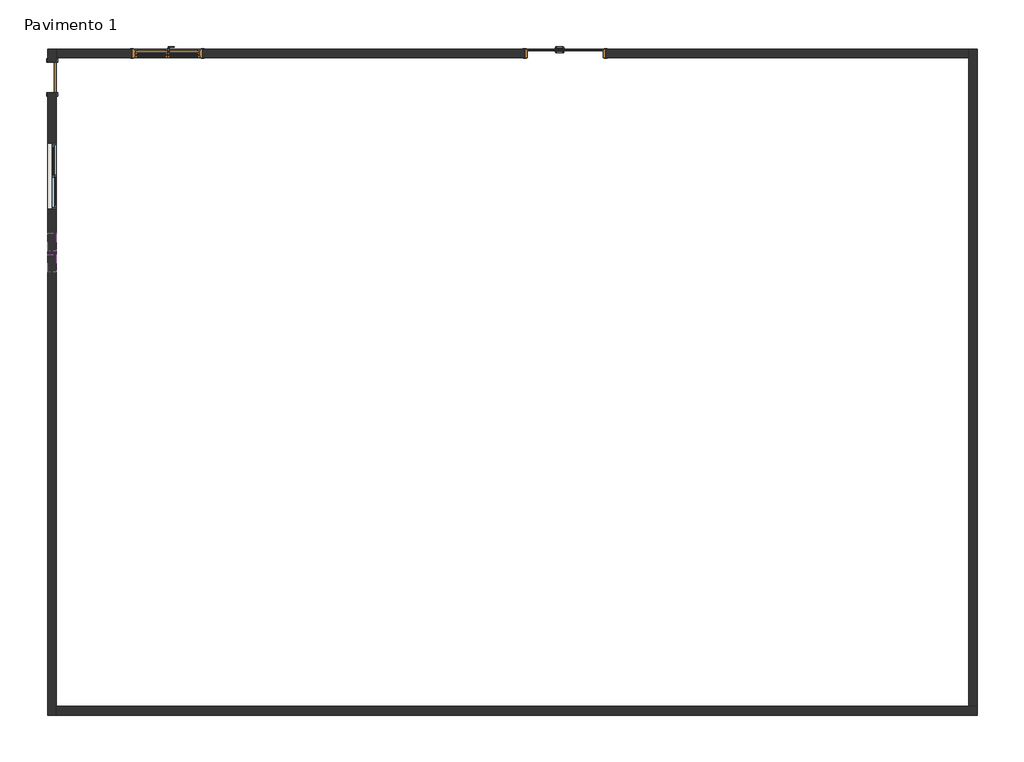
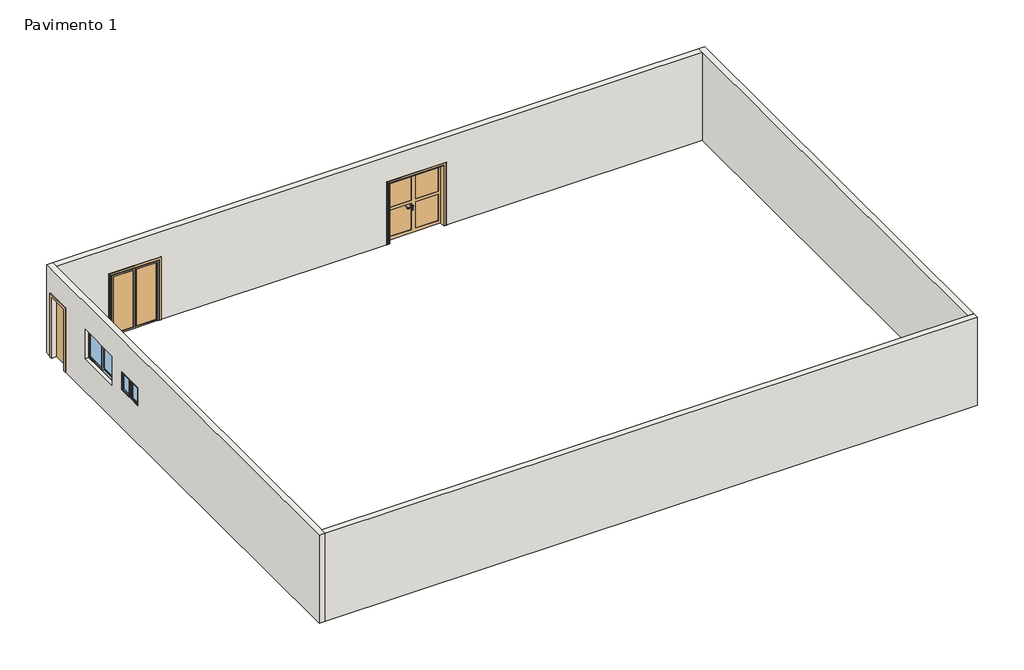
# One storey: 4 walls, 3 doors, 3 windows.
# Revit data of these elements (continued)
# Type "Abertura da porta e vidraça com revestimento : .Porta 160x210" (continued)
#   Analytic Construction = "Metal"
#   W1 = 0.046 m
#   Largura da apara = 0.07 m
#   Espessura da apara = 0.01 m
#   Rough Width = 1.60 m
#   Rough Height = 2.10 m
#   Largura da moldura do painel = 0.05 m
#   Espessura da moldura do painel = 0.04 m
#   Heat Transfer Coefficient (U) = 3.7021 W/(m²·K)
#   Height = 2.10 m
#   Width = 1.60 m
#   Largura da estrutura = 0.05 m
#   Define Thermal Properties by = 1
#   Function = 1
#   Material da apara = Aço inoxidável
#   Material do painel = Vidro
#   Material do puxador = Aço inoxidável
#   Vidro = Vidro
#   Material da moldura = Aço inoxidável
#   Visual Light Transmittance = 0
#   Solar Heat Gain Coefficient = 0
#   Wall Closure = (empty or 0)
# Type "Porta de entrada dupla com revestimento : 1840 x 2100mm"
#   Type Mark = "46"
#   Construction Type Id = "MDOOR"
#   Analytic Construction = "Metal"
#   W2 = 0.92 m
#   W1 = 1.76 m
#   Largura da apara = 0.07 m
#   Espessura da apara = 0.008 m
#   Thickness = 0.035 m
#   Rough Width = 1.84 m
#   Rough Height = 2.10 m
#   Largura da moldura do painel = 0.075 m
#   Heat Transfer Coefficient (U) = 3.7021 W/(m²·K)
#   Largura da estrutura = 0.05 m
#   Height = 2.10 m
#   Width = 1.84 m
#   Define Thermal Properties by = 1
#   Function = 1
#   Material da apara = none
#   Material do painel = none
#   Material do puxador = none
#   Vidro = none
#   Material da moldura = none
#   Visual Light Transmittance = 0
#   Solar Heat Gain Coefficient = 0
#   Wall Closure = (empty or 0)
# Type ".Parede 020 cm"
#   Layers, outside or top first: 0.01 m ".Tinta externa branco gelo" (function 4); 0.03 m ".Revestimento de concreto" (function 4); 0.12 m ".Tijolo 9 cm" (function 1); 0.03 m ".Revestimento de concreto" (function 4); 0.01 m ".Tinta externa branco gelo" (function 4)
# Type "Janela de correr - 2 Painéis : .Janela 2 Folhas - 150x100/110"
#   Type Mark = "20"
#   Construction Type Id = "GSP4R"
#   Analytic Construction = "Vidraça única Pilkington 1/8 pol"
#   Visual Light Transmittance = 0.9
#   Solar Heat Gain Coefficient = 0.78
#   Rough Width = 1.50 m
#   Rough Height = 1.00 m
#   Largura da moldura do painel = 0.05 m
#   Espessura da moldura do painel = 0.04 m
#   Height = 1.00 m
#   Heat Transfer Coefficient (U) = 3.6886 W/(m²·K)
#   Largura da estrutura = 0.035 m
#   Espessura da moldura = 0.09 m
#   Altura-padrão do peitoril = 1.10 m
#   Width = 1.50 m
#   Define Thermal Properties by = 1
#   Vidro = none
#   Material da moldura = none
#   Wall Closure = (empty or 0)
# Type "M_Fixo : 0406 x 0610mm"
#   Type Mark = "10"
#   Construction Type Id = "GSP4R"
#   Analytic Construction = "Vidraça única Pilkington 1/8 pol"
#   Visual Light Transmittance = 0.9
#   Thermal Resistance (R) = 0.271106 (m²·K)/W
#   Solar Heat Gain Coefficient = 0.78
#   Heat Transfer Coefficient (U) = 3.6886 W/(m²·K)
#   Height = 0.61 m
#   Altura-padrão do peitoril = 0.915 m
#   Width = 0.406 m
#   Janela aplicada = 0.019 m
#   Define Thermal Properties by = 1
#   Material da estrutura externa = Caixilho
#   Material da estrutura interna = Caixilho
#   Material do painel de vidro = Vidro
#   Caixilho = Caixilho
#   Wall Closure = (empty or 0)
# Element 1 (IfcDoor, "M_Folha única : .Porta - 210x070")
#   Phase Created = Construção nova
#   Materials on its faces: "Porta - Batente", "Porta - Painel"
# Element 2 (IfcDoor, "Abertura da porta e vidraça com revestimento : .Porta 160x210")
#   Phase Created = Construção nova
#   Materials on its faces: "Aço inoxidável", "Vidro"
# Element 3 (IfcDoor, "Porta de entrada dupla com revestimento : 1840 x 2100mm")
#   Phase Created = Construção nova
#   Materials on its faces: "Vidro"
# Element 4 (IfcWall, ".Parede 020 cm")
#   Top Offset = 0.00 m
#   Base Offset = 0.00 m
#   wall height = 3.00 m
#   Phase Created = Construção nova
#   Base Constraint = Pavimento 1
#   Top Constraint = Pavimento 2
#   Materials on its faces: "Material pré-definido de parede", ".Tinta bege", ".Tinta externa branco gelo"
# Element 5 (IfcWall, ".Parede 020 cm")
#   Top Offset = 0.00 m
#   Base Offset = 0.00 m
#   wall height = 3.00 m
#   Phase Created = Construção nova
#   Base Constraint = Pavimento 1
#   Top Constraint = Pavimento 2
#   Materials on its faces: ".Tinta bege", ".Tinta externa branco gelo", "Material pré-definido de parede"
# Element 6 (IfcWall, ".Parede 020 cm")
#   Top Offset = 0.00 m
#   Base Offset = 0.00 m
#   wall height = 3.00 m
#   Phase Created = Construção nova
#   Base Constraint = Pavimento 1
#   Top Constraint = Pavimento 2
#   Materials on its faces: ".Tinta bege", "Material pré-definido de parede", ".Tinta externa branco gelo"
# Element 7 (IfcWall, ".Parede 020 cm")
#   Top Offset = 0.00 m
#   Base Offset = 0.00 m
#   wall height = 3.00 m
#   Phase Created = Construção nova
#   Base Constraint = Pavimento 1
#   Top Constraint = Pavimento 2
#   Materials on its faces: "Material pré-definido de parede", ".Tinta externa branco gelo"
# Element 8 (IfcWindow, "Janela de correr - 2 Painéis : .Janela 2 Folhas - 150x100/110")
#   Mark = "3"
#   Phase Created = Construção nova
#   Materials on its faces: "Vidro"
# Element 9 (IfcWindow, "M_Fixo : 0406 x 0610mm")
#   Mark = "1"
#   Phase Created = Construção nova
#   Materials on its faces: "Caixilho", "Vidro"
# Element 10 (IfcWindow, "M_Fixo : 0406 x 0610mm")
#   Mark = "2"
#   Phase Created = Construção nova
#   Materials on its faces: "Caixilho", "Vidro"
# Materials
#   "Porta - Painel": class "Madeira", colour RGB 210 159 95, transparency 0, Cost = 0
#   "Porta - Batente": class "Diversos", colour RGB 118 70 51, transparency 0, Cost = 0
#   "Aço inoxidável": class "Metal", colour RGB 0 0 0, transparency 0, Description = "Aço inoxidável 18/8", Cost = 0
#   "Vidro": class "Vidro", colour RGB 0 128 192, transparency 0.9, Description = "Vidro de sílica", Cost = 0
#   ".Tinta externa branco gelo": class "Genérico", colour RGB 210 210 210, transparency 0, Cost = 0
#   ".Revestimento de concreto": class "Genérico", colour RGB 120 120 120, transparency 0, Cost = 0
#   ".Tijolo 9 cm": class "Genérico", colour RGB 255 255 255, transparency 0, Cost = 0
#   "Caixilho": class "Madeira", colour RGB 224 178 126, transparency 0, Cost = 0
#   "Material pré-definido de parede": class "Diversos", colour RGB 128 128 128, transparency 0, Cost = 0
#   ".Tinta bege": class "Genérico", colour RGB 245 245 245, transparency 0, Cost = 0
